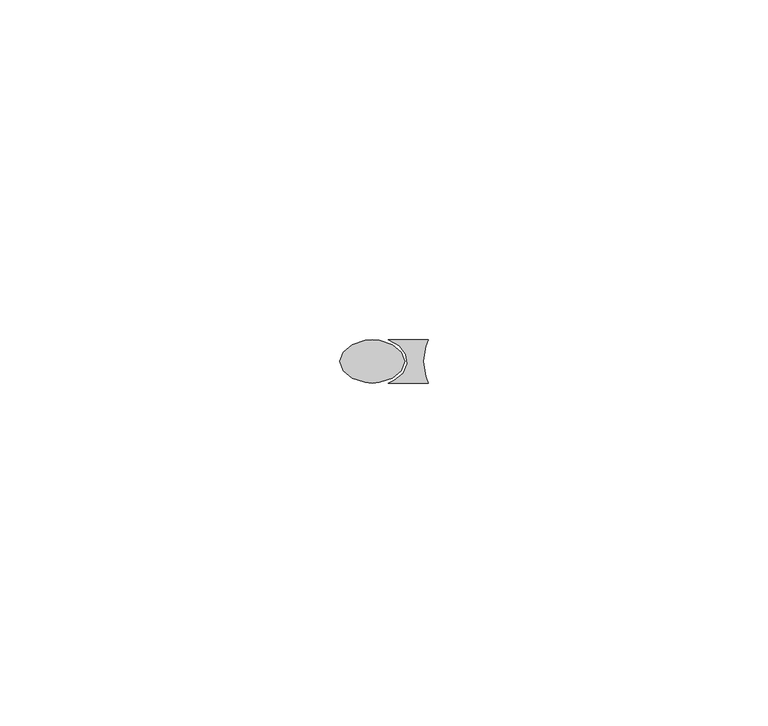
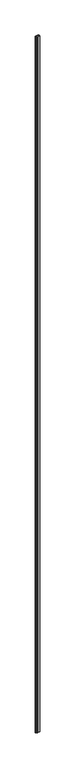
"""IFC4 building model written with IfcOpenShell, lengths in millimetres: proxy geometry, Generic Models 11:Generic Models 1:306267:Generic Models 1:306267 : Generic Models 11:Generic Models 1:306267:300405:Generic Models 1:306267:Generic Models 1:306267 : Generic Models 11:Generic Models 1:306267:300405 : Generic Models 11:Generic Models 1:306267:Generic Models 1:306267 : Generic Models 11:Generic Models 1:306267:300405:15 : Generic Models 11:Generic Models 1:306267:Generic Models 1:306267 : Generic Models 11:Generic Models 1:306267:300405:Generic Models 1:306267:Generic Models 1:306267 : Generic Models 11:Generic Models 1:306267:300405 : Generic Models 11:Generic Models 1:306267:Generic Models 1:306267 : Generic Models 11:Generic Models 1:306267:300405:300182."""

from ifc_helpers import new_model, si_unit, origin, origin_with_axes, place, context, project, spatial, polyline, outline, extrude, source, transform, mapped, element, save


def generic_models_fef91386(model_context):
    return source(origin(), model_context, "Body", "SweptSolid", [
        extrude(outline(polyline([(573367.5409469, -536525.0496088), (573366.2194528, -536526.1543429), (573364.3098386, -536526.7674241), (573363.2500826, -536526.8470279), (573362.1903267, -536526.7674241), (573360.2807125, -536526.1543429), (573358.9592184, -536525.0496088), (573358.4875826, -536523.6720279), (573358.9592184, -536522.2944471), (573360.2807125, -536521.189713), (573362.1903267, -536520.5766318), (573363.2500826, -536520.4970279), (573364.3098386, -536520.5766318), (573366.2194528, -536521.189713), (573367.5409469, -536522.2944471), (573368.0125826, -536523.6720279), (573367.5409469, -536525.0496088)])), origin_with_axes(), (0.0, 0.0, 1.0), 2495.55),
        extrude(outline(polyline([(573371.1043937, -536521.4627912), (573370.7907076, -536523.6720279), (573371.1043937, -536525.8812647), (573371.4818023, -536526.8470279), (573365.6137102, -536526.8470279), (573366.4739912, -536526.4607104), (573367.7835663, -536525.3772249), (573368.3839199, -536524.0269772), (573368.181132, -536522.6212009), (573367.206927, -536521.3798168), (573365.6137102, -536520.4970279), (573371.4818023, -536520.4970279), (573371.1043937, -536521.4627912)])), origin_with_axes(), (0.0, 0.0, 1.0), 2495.55),
    ])


if __name__ == "__main__":
    model = new_model("IFC4")
    model_context = context("Model", 3, world=origin())
    ifc_project = project(units=[si_unit("LENGTHUNIT", "METRE", prefix="MILLI")], contexts=[model_context])
    site = spatial("IfcSite", under=ifc_project)
    building = spatial("IfcBuilding", under=site)
    placement = place(None, origin())
    generic_models_shape = generic_models_fef91386(model_context)
    element("IfcBuildingElementProxy", 1, Name="Generic Models 11:Generic Models 1:306267:Generic Models 1:306267 : Generic Models 11:Generic Models 1:306267:300405:Generic Models 1:306267:Generic Models 1:306267 : Generic Models 11:Generic Models 1:306267:300405 : Generic Models 11:Generic Models 1:306267:Generic Models 1:306267 : Generic Models 11:Generic Models 1:306267:300405:15 : Generic Models 11:Generic Models 1:306267:Generic Models 1:306267 : Generic Models 11:Generic Models 1:306267:300405:Generic Models 1:306267:Generic Models 1:306267 : Generic Models 11:Generic Models 1:306267:300405 : Generic Models 11:Generic Models 1:306267:Generic Models 1:306267 : Generic Models 11:Generic Models 1:306267:300405:300182", ObjectType="Generic Models 11:Generic Models 1:306267:Generic Models 1:306267 : Generic Models 11:Generic Models 1:306267:300405:Generic Models 1:306267:Generic Models 1:306267 : Generic Models 11:Generic Models 1:306267:300405 : Generic Models 11:Generic Models 1:306267:Generic Models 1:306267 : Generic Models 11:Generic Models 1:306267:300405:15 : Generic Models 11:Generic Models 1:306267:Generic Models 1:306267 : Generic Models 11:Generic Models 1:306267:300405:Generic Models 1:306267:Generic Models 1:306267 : Generic Models 11:Generic Models 1:306267:300405 : Generic Models 11:Generic Models 1:306267:Generic Models 1:306267 : Generic Models 11:Generic Models 1:306267:300405:300182", at=placement, inside=building, context=model_context, shape_type="MappedRepresentation", body=[
        mapped(generic_models_shape, transform((0.0, 0.0, 0.0), x_axis=(1.0, 0.0, 0.0), y_axis=(0.0, 1.0, 0.0), z_axis=(0.0, 0.0, 1.0))),
    ])
    save(model, "model.ifc")

# Revit data of these elements
# Type "Generic Models 11:Generic Models 1:306267:Generic Models 1:306267 : Generic Models 11:Generic Models 1:306267:300405:Generic Models 1:306267:Generic Models 1:306267 : Generic Models 11:Generic Models 1:306267:300405 : Generic Models 11:Generic Models 1:306267:Generic Models 1:306267 : Generic Models 11:Generic Models 1:306267:300405:15 : Generic Models 11:Generic Models 1:306267:Generic Models 1:306267 : Generic Models 11:Generic Models 1:306267:300405:Generic Models 1:306267:Generic Models 1:306267 : Generic Models 11:Generic Models 1:306267:300405 : Generic Models 11:Generic Models 1:306267:Generic Models 1:306267 : Generic Models 11:Generic Models 1:306267:300405:300182"
#   NameOverride = "Generic Models 11:Generic Models 1:306267:Generic Models 1:306267 : Generic Models 11:Generic Models 1:306267:300405:Generic Models 1:306267:Generic Models 1:306267 : Generic Models 11:Generic Models 1:306267:300405 : Generic Models 11:Generic Models 1:306267:Generic Models 1:306267 : Generic Models 11:Generic Models 1:306267:300405:300182"
#   ObjectTypeOverride = "Generic Models 1:306267:Generic Models 1:306267 : Generic Models 11:Generic Models 1:306267:300405 : Generic Models 11:Generic Models 1:306267:Generic Models 1:306267 : Generic Models 11:Generic Models 1:306267:300405"
#   Reference = "Generic Models 1"
#   Tag = "300182"
# Element 1 (IfcBuildingElementProxy, "Generic Models 11:Generic Models 1:306267:Generic Models 1:306267 : Generic Models 11:Generic Models 1:306267:300405:Generic Models 1:306267:Generic Models 1:306267 : Generic Models 11:Generic Models 1:306267:300405 : Generic Models 11:Generic Models 1:306267:Generic Models 1:306267 : Generic Models 11:Generic Models 1:306267:300405:15 : Generic Models 11:Generic Models 1:306267:Generic Models 1:306267 : Generic Models 11:Generic Models 1:306267:300405:Generic Models 1:306267:Generic Models 1:306267 : Generic Models 11:Generic Models 1:306267:300405 : Generic Models 11:Generic Models 1:306267:Generic Models 1:306267 : Generic Models 11:Generic Models 1:306267:300405:300182")
#   Materials on its faces: "SEALANT & BACKER ROD, IF NECESSARY"
# Materials
#   "SEALANT & BACKER ROD, IF NECESSARY": class "Unassigned", colour RGB 120 120 120, transparency 0, Cost = 0
